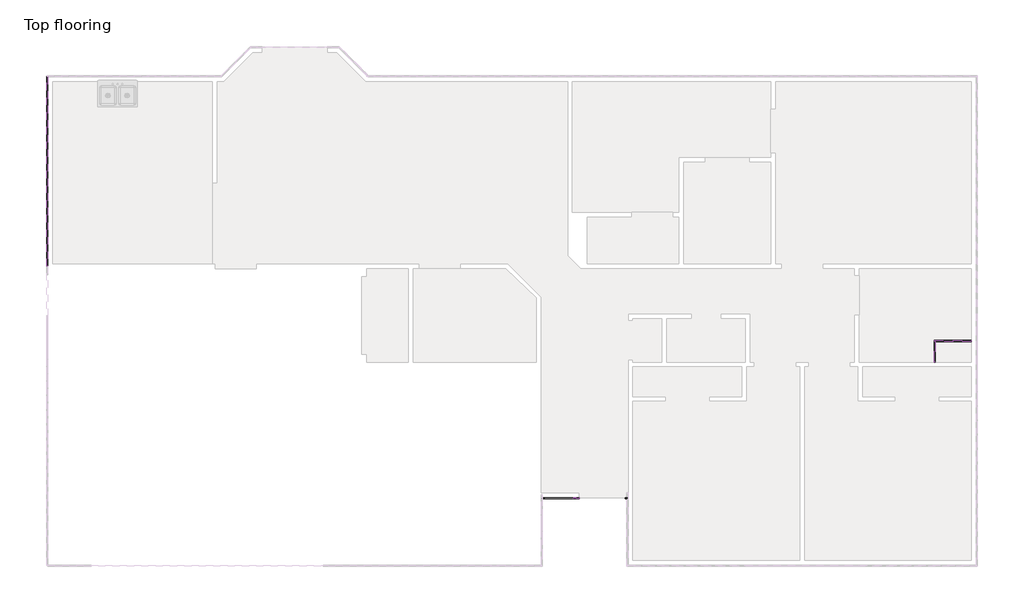
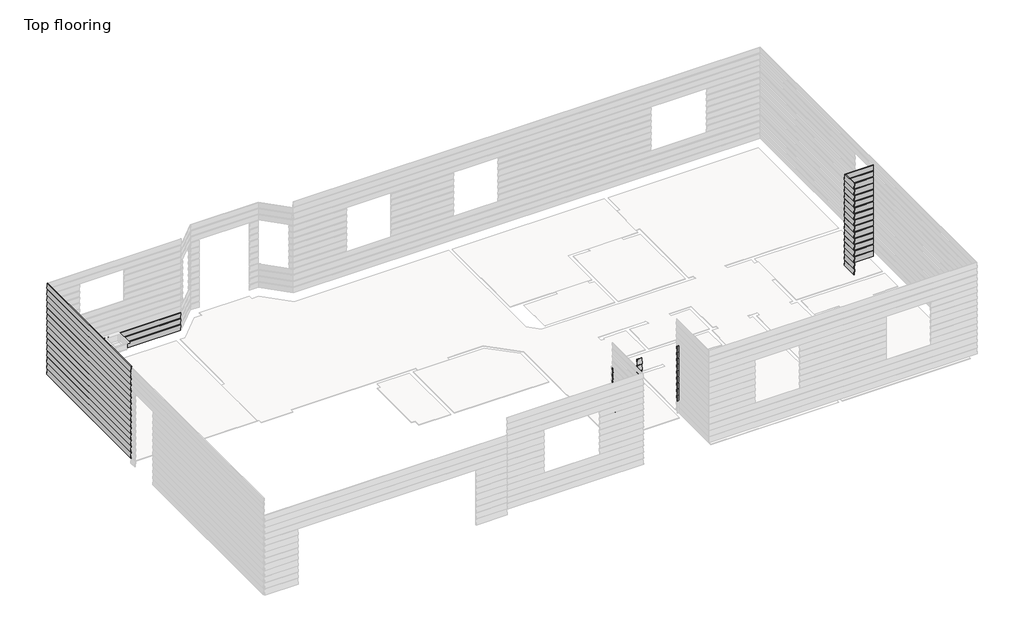
# One storey, part 3 of 5: 57 proxies.
"""IFC4 building model written with IfcOpenShell, lengths in millimetres."""

from ifc_helpers import new_model, si_unit, frame, origin, place, context, project, spatial, polyline, outline, extrude, faceted_brep, element, save

model = new_model("IFC4")

# Units and contexts
model_context = context("Model", 3, world=origin())
ifc_project = project(units=[si_unit("LENGTHUNIT", "METRE", prefix="MILLI")], contexts=[model_context])

# Site, building, storey
site = spatial("IfcSite", under=ifc_project)
building = spatial("IfcBuilding", under=site)
storey = spatial("IfcBuildingStorey", under=building, Name="Top flooring", Elevation=12.7)

# Proxies
placement = place(None, origin())
element("IfcBuildingElementProxy", 1, Name="Wall Sweeps", at=placement, inside=storey, context=model_context, shape_type="Brep", body=[
    faceted_brep([(-17825.3509195, 5231.8645018, 179.3151454), (-17811.1755052, 5217.6890875, 338.6859634), (-17801.214829, 5207.7284114, 337.8), (-17815.3902433, 5221.9038257, 178.429182), (-17825.3509195, 1226.2784114, 179.3151454), (-17815.3902433, 1226.2784114, 178.429182), (-17801.214829, 1226.2784114, 337.8), (-17811.1755052, 1226.2784114, 338.6859634)], [[[0, 1, 2, 3]], [[4, 5, 6, 7]], [[1, 0, 4, 7]], [[2, 1, 7, 6]], [[3, 2, 6, 5]], [[0, 3, 5, 4]]]),
])
element("IfcBuildingElementProxy", 2, Name="Wall Sweeps", at=placement, inside=storey, context=model_context, shape_type="Brep", body=[
    faceted_brep([(-17825.3509195, 5231.8645018, 357.1151454), (-17811.1755052, 5217.6890875, 516.4859634), (-17801.214829, 5207.7284114, 515.6), (-17815.3902433, 5221.9038257, 356.229182), (-17825.3509195, 1226.2784114, 357.1151454), (-17815.3902433, 1226.2784114, 356.229182), (-17801.214829, 1226.2784114, 515.6), (-17811.1755052, 1226.2784114, 516.4859634)], [[[0, 1, 2, 3]], [[4, 5, 6, 7]], [[1, 0, 4, 7]], [[2, 1, 7, 6]], [[3, 2, 6, 5]], [[0, 3, 5, 4]]]),
])
element("IfcBuildingElementProxy", 3, Name="Wall Sweeps", at=placement, inside=storey, context=model_context, shape_type="Brep", body=[
    faceted_brep([(-17825.3509195, 5231.8645018, 534.9151454), (-17811.1755052, 5217.6890875, 694.2859634), (-17801.214829, 5207.7284114, 693.4), (-17815.3902433, 5221.9038257, 534.029182), (-17825.3509195, 1226.2784114, 534.9151454), (-17815.3902433, 1226.2784114, 534.029182), (-17801.214829, 1226.2784114, 693.4), (-17811.1755052, 1226.2784114, 694.2859634)], [[[0, 1, 2, 3]], [[4, 5, 6, 7]], [[1, 0, 4, 7]], [[2, 1, 7, 6]], [[3, 2, 6, 5]], [[0, 3, 5, 4]]]),
])
element("IfcBuildingElementProxy", 4, Name="Wall Sweeps", at=placement, inside=storey, context=model_context, shape_type="Brep", body=[
    faceted_brep([(-17825.3509195, 5231.8645018, 712.7151454), (-17811.1755052, 5217.6890875, 872.0859634), (-17801.214829, 5207.7284114, 871.2), (-17815.3902433, 5221.9038257, 711.829182), (-17825.3509195, 1226.2784114, 712.7151454), (-17815.3902433, 1226.2784114, 711.829182), (-17801.214829, 1226.2784114, 871.2), (-17811.1755052, 1226.2784114, 872.0859634)], [[[0, 1, 2, 3]], [[4, 5, 6, 7]], [[1, 0, 4, 7]], [[2, 1, 7, 6]], [[3, 2, 6, 5]], [[0, 3, 5, 4]]]),
])
element("IfcBuildingElementProxy", 5, Name="Wall Sweeps", at=placement, inside=storey, context=model_context, shape_type="Brep", body=[
    faceted_brep([(-17825.3509195, 5231.8645018, 890.5151454), (-17811.1755052, 5217.6890875, 1049.8859634), (-17801.214829, 5207.7284114, 1049.0), (-17815.3902433, 5221.9038257, 889.629182), (-17825.3509195, 1226.2784114, 890.5151454), (-17815.3902433, 1226.2784114, 889.629182), (-17801.214829, 1226.2784114, 1049.0), (-17811.1755052, 1226.2784114, 1049.8859634)], [[[0, 1, 2, 3]], [[4, 5, 6, 7]], [[1, 0, 4, 7]], [[2, 1, 7, 6]], [[3, 2, 6, 5]], [[0, 3, 5, 4]]]),
])
element("IfcBuildingElementProxy", 6, Name="Wall Sweeps", at=placement, inside=storey, context=model_context, shape_type="Brep", body=[
    faceted_brep([(-17825.3509195, 5231.8645018, 1068.3151454), (-17811.1755052, 5217.6890875, 1227.6859634), (-17801.214829, 5207.7284114, 1226.8), (-17815.3902433, 5221.9038257, 1067.429182), (-17825.3509195, 1226.2784114, 1068.3151454), (-17815.3902433, 1226.2784114, 1067.429182), (-17801.214829, 1226.2784114, 1226.8), (-17811.1755052, 1226.2784114, 1227.6859634)], [[[0, 1, 2, 3]], [[4, 5, 6, 7]], [[1, 0, 4, 7]], [[2, 1, 7, 6]], [[3, 2, 6, 5]], [[0, 3, 5, 4]]]),
])
element("IfcBuildingElementProxy", 7, Name="Wall Sweeps", at=placement, inside=storey, context=model_context, shape_type="Brep", body=[
    faceted_brep([(-17825.3509195, 5231.8645018, 1246.1151454), (-17811.1755052, 5217.6890875, 1405.4859634), (-17801.214829, 5207.7284114, 1404.6), (-17815.3902433, 5221.9038257, 1245.229182), (-17825.3509195, 1226.2784114, 1246.1151454), (-17815.3902433, 1226.2784114, 1245.229182), (-17801.214829, 1226.2784114, 1404.6), (-17811.1755052, 1226.2784114, 1405.4859634)], [[[0, 1, 2, 3]], [[4, 5, 6, 7]], [[1, 0, 4, 7]], [[2, 1, 7, 6]], [[3, 2, 6, 5]], [[0, 3, 5, 4]]]),
])
element("IfcBuildingElementProxy", 8, Name="Wall Sweeps", at=placement, inside=storey, context=model_context, shape_type="Brep", body=[
    faceted_brep([(-17825.3509195, 5231.8645018, 1423.9151454), (-17811.1755052, 5217.6890875, 1583.2859634), (-17801.214829, 5207.7284114, 1582.4), (-17815.3902433, 5221.9038257, 1423.029182), (-17825.3509195, 1226.2784114, 1423.9151454), (-17815.3902433, 1226.2784114, 1423.029182), (-17801.214829, 1226.2784114, 1582.4), (-17811.1755052, 1226.2784114, 1583.2859634)], [[[0, 1, 2, 3]], [[4, 5, 6, 7]], [[1, 0, 4, 7]], [[2, 1, 7, 6]], [[3, 2, 6, 5]], [[0, 3, 5, 4]]]),
])
element("IfcBuildingElementProxy", 9, Name="Wall Sweeps", at=placement, inside=storey, context=model_context, shape_type="Brep", body=[
    faceted_brep([(-17825.3509195, 5231.8645018, 1601.7151454), (-17811.1755052, 5217.6890875, 1761.0859634), (-17801.214829, 5207.7284114, 1760.2), (-17815.3902433, 5221.9038257, 1600.829182), (-17825.3509195, 1226.2784114, 1601.7151454), (-17815.3902433, 1226.2784114, 1600.829182), (-17801.214829, 1226.2784114, 1760.2), (-17811.1755052, 1226.2784114, 1761.0859634)], [[[0, 1, 2, 3]], [[4, 5, 6, 7]], [[1, 0, 4, 7]], [[2, 1, 7, 6]], [[3, 2, 6, 5]], [[0, 3, 5, 4]]]),
])
element("IfcBuildingElementProxy", 10, Name="Wall Sweeps", at=placement, inside=storey, context=model_context, shape_type="Brep", body=[
    faceted_brep([(-17825.3509195, 5231.8645018, 1779.5151454), (-17811.1755052, 5217.6890875, 1938.8859634), (-17801.214829, 5207.7284114, 1938.0), (-17815.3902433, 5221.9038257, 1778.629182), (-17825.3509195, 1226.2784114, 1779.5151454), (-17815.3902433, 1226.2784114, 1778.629182), (-17801.214829, 1226.2784114, 1938.0), (-17811.1755052, 1226.2784114, 1938.8859634)], [[[0, 1, 2, 3]], [[4, 5, 6, 7]], [[1, 0, 4, 7]], [[2, 1, 7, 6]], [[3, 2, 6, 5]], [[0, 3, 5, 4]]]),
])
element("IfcBuildingElementProxy", 11, Name="Wall Sweeps", at=placement, inside=storey, context=model_context, shape_type="Brep", body=[
    faceted_brep([(-17825.3509195, 5231.8645018, 1957.3151454), (-17811.1755052, 5217.6890875, 2116.6859634), (-17801.214829, 5207.7284114, 2115.8), (-17815.3902433, 5221.9038257, 1956.429182), (-17825.3509195, 1226.2784114, 1957.3151454), (-17815.3902433, 1226.2784114, 1956.429182), (-17801.214829, 1226.2784114, 2115.8), (-17811.1755052, 1226.2784114, 2116.6859634)], [[[0, 1, 2, 3]], [[4, 5, 6, 7]], [[1, 0, 4, 7]], [[2, 1, 7, 6]], [[3, 2, 6, 5]], [[0, 3, 5, 4]]]),
])
element("IfcBuildingElementProxy", 12, Name="Wall Sweeps", at=placement, inside=storey, context=model_context, shape_type="Brep", body=[
    faceted_brep([(-17825.3509195, 5231.8645018, 2135.1151454), (-17811.1755052, 5217.6890875, 2294.4859634), (-17801.214829, 5207.7284114, 2293.6), (-17815.3902433, 5221.9038257, 2134.229182), (-17825.3509195, 1226.2784114, 2135.1151454), (-17815.3902433, 1226.2784114, 2134.229182), (-17801.214829, 1226.2784114, 2293.6), (-17811.1755052, 1226.2784114, 2294.4859634)], [[[0, 1, 2, 3]], [[4, 5, 6, 7]], [[1, 0, 4, 7]], [[2, 1, 7, 6]], [[3, 2, 6, 5]], [[0, 3, 5, 4]]]),
])
element("IfcBuildingElementProxy", 13, Name="Wall Sweeps", at=placement, inside=storey, context=model_context, shape_type="Brep", body=[
    faceted_brep([(-17825.3509195, 5231.8645018, 179.3151454), (-17815.3902433, 5221.9038257, 178.429182), (-17801.214829, 5207.7284114, 337.8), (-17811.1755052, 5217.6890875, 338.6859634), (-14153.612325, 5231.8645018, 179.3151454), (-14147.7406762, 5217.6890875, 338.6859634), (-14143.614829, 5207.7284114, 337.8), (-14149.4864779, 5221.9038257, 178.429182)], [[[0, 1, 2, 3]], [[4, 5, 6, 7]], [[1, 0, 4, 7]], [[2, 1, 7, 6]], [[3, 2, 6, 5]], [[0, 3, 5, 4]]]),
])
element("IfcBuildingElementProxy", 14, Name="Wall Sweeps", at=placement, inside=storey, context=model_context, shape_type="Brep", body=[
    faceted_brep([(-17825.3509195, 5231.8645018, 357.1151454), (-17815.3902433, 5221.9038257, 356.229182), (-17801.214829, 5207.7284114, 515.6), (-17811.1755052, 5217.6890875, 516.4859634), (-14153.612325, 5231.8645018, 357.1151454), (-14147.7406762, 5217.6890875, 516.4859634), (-14143.614829, 5207.7284114, 515.6), (-14149.4864779, 5221.9038257, 356.229182)], [[[0, 1, 2, 3]], [[4, 5, 6, 7]], [[1, 0, 4, 7]], [[2, 1, 7, 6]], [[3, 2, 6, 5]], [[0, 3, 5, 4]]]),
])
element("IfcBuildingElementProxy", 15, Name="Wall Sweeps", at=placement, inside=storey, context=model_context, shape_type="Brep", body=[
    faceted_brep([(-17825.3509195, 5231.8645018, 534.9151454), (-17815.3902433, 5221.9038257, 534.029182), (-17801.214829, 5207.7284114, 693.4), (-17811.1755052, 5217.6890875, 694.2859634), (-14153.612325, 5231.8645018, 534.9151454), (-14147.7406762, 5217.6890875, 694.2859634), (-14143.614829, 5207.7284114, 693.4), (-14149.4864779, 5221.9038257, 534.029182)], [[[0, 1, 2, 3]], [[4, 5, 6, 7]], [[1, 0, 4, 7]], [[2, 1, 7, 6]], [[3, 2, 6, 5]], [[0, 3, 5, 4]]]),
])
element("IfcBuildingElementProxy", 16, Name="Wall Sweeps", at=placement, inside=storey, context=model_context, shape_type="SweptSolid", body=[
    extrude(outline(polyline([(0.0, -10.0), (0.0, 0.0), (63.9, 0.0), (63.9, -10.0), (0.0, -10.0)])), frame((-5673.114829, -3645.6470029, 534.029182), z_axis=(0.0, 0.08859633935570814, 0.9960676124906221), x_axis=(1.0, 0.0, 0.0)), (0.0, 0.0, 1.0), 160.0),
    extrude(outline(polyline([(0.0, -10.0), (0.0, 0.0), (800.5, 0.0), (800.5, -10.0), (0.0, -10.0)])), frame((-7438.014829, -3645.6470029, 534.029182), z_axis=(0.0, 0.08859633935570814, 0.9960676124906221), x_axis=(1.0, 0.0, 0.0)), (0.0, 0.0, 1.0), 160.0),
])
element("IfcBuildingElementProxy", 17, Name="Wall Sweeps", at=placement, inside=storey, context=model_context, shape_type="SweptSolid", body=[
    extrude(outline(polyline([(0.0, -10.0), (0.0, 0.0), (63.9, 0.0), (63.9, -10.0), (0.0, -10.0)])), frame((-5673.114829, -3645.6470029, 711.829182), z_axis=(0.0, 0.08859633935570814, 0.9960676124906221), x_axis=(1.0, 0.0, 0.0)), (0.0, 0.0, 1.0), 160.0),
    extrude(outline(polyline([(0.0, -10.0), (0.0, 0.0), (800.5, 0.0), (800.5, -10.0), (0.0, -10.0)])), frame((-7438.014829, -3645.6470029, 711.829182), z_axis=(0.0, 0.08859633935570814, 0.9960676124906221), x_axis=(1.0, 0.0, 0.0)), (0.0, 0.0, 1.0), 160.0),
])
element("IfcBuildingElementProxy", 18, Name="Wall Sweeps", at=placement, inside=storey, context=model_context, shape_type="SweptSolid", body=[
    extrude(outline(polyline([(0.0, -10.0), (0.0, 0.0), (63.9, 0.0), (63.9, -10.0), (0.0, -10.0)])), frame((-5673.114829, -3645.6470029, 889.629182), z_axis=(0.0, 0.08859633935570814, 0.9960676124906221), x_axis=(1.0, 0.0, 0.0)), (0.0, 0.0, 1.0), 160.0),
    extrude(outline(polyline([(0.0, -10.0), (0.0, 0.0), (127.4, 0.0), (127.4, -10.0), (0.0, -10.0)])), frame((-6764.914829, -3645.6470029, 889.629182), z_axis=(0.0, 0.08859633935570814, 0.9960676124906221), x_axis=(1.0, 0.0, 0.0)), (0.0, 0.0, 1.0), 160.0),
    extrude(outline(polyline([(0.0, -10.0), (0.0, 0.0), (63.5, 0.0), (63.5, -10.0), (0.0, -10.0)])), frame((-7438.014829, -3645.6470029, 889.629182), z_axis=(0.0, 0.08859633935570814, 0.9960676124906221), x_axis=(1.0, 0.0, 0.0)), (0.0, 0.0, 1.0), 160.0),
])
element("IfcBuildingElementProxy", 19, Name="Wall Sweeps", at=placement, inside=storey, context=model_context, shape_type="SweptSolid", body=[
    extrude(outline(polyline([(0.0, -10.0), (0.0, 0.0), (63.9, 0.0), (63.9, -10.0), (0.0, -10.0)])), frame((-5673.114829, -3645.6470029, 1067.429182), z_axis=(0.0, 0.08859633935570814, 0.9960676124906221), x_axis=(1.0, 0.0, 0.0)), (0.0, 0.0, 1.0), 160.0),
    extrude(outline(polyline([(0.0, -10.0), (0.0, 0.0), (127.4, 0.0), (127.4, -10.0), (0.0, -10.0)])), frame((-6764.914829, -3645.6470029, 1067.429182), z_axis=(0.0, 0.08859633935570814, 0.9960676124906221), x_axis=(1.0, 0.0, 0.0)), (0.0, 0.0, 1.0), 160.0),
    extrude(outline(polyline([(0.0, -10.0), (0.0, 0.0), (63.5, 0.0), (63.5, -10.0), (0.0, -10.0)])), frame((-7438.014829, -3645.6470029, 1067.429182), z_axis=(0.0, 0.08859633935570814, 0.9960676124906221), x_axis=(1.0, 0.0, 0.0)), (0.0, 0.0, 1.0), 160.0),
])
element("IfcBuildingElementProxy", 20, Name="Wall Sweeps", at=placement, inside=storey, context=model_context, shape_type="SweptSolid", body=[
    extrude(outline(polyline([(0.0, -10.0), (0.0, 0.0), (63.9, 0.0), (63.9, -10.0), (0.0, -10.0)])), frame((-5673.114829, -3645.6470029, 1245.229182), z_axis=(0.0, 0.08859633935570814, 0.9960676124906221), x_axis=(1.0, 0.0, 0.0)), (0.0, 0.0, 1.0), 160.0),
    extrude(outline(polyline([(0.0, -10.0), (0.0, 0.0), (127.4, 0.0), (127.4, -10.0), (0.0, -10.0)])), frame((-6764.914829, -3645.6470029, 1245.229182), z_axis=(0.0, 0.08859633935570814, 0.9960676124906221), x_axis=(1.0, 0.0, 0.0)), (0.0, 0.0, 1.0), 160.0),
    extrude(outline(polyline([(0.0, -10.0), (0.0, 0.0), (63.5, 0.0), (63.5, -10.0), (0.0, -10.0)])), frame((-7438.014829, -3645.6470029, 1245.229182), z_axis=(0.0, 0.08859633935570814, 0.9960676124906221), x_axis=(1.0, 0.0, 0.0)), (0.0, 0.0, 1.0), 160.0),
])
element("IfcBuildingElementProxy", 21, Name="Wall Sweeps", at=placement, inside=storey, context=model_context, shape_type="SweptSolid", body=[
    extrude(outline(polyline([(0.0, -10.0), (0.0, 0.0), (63.9, 0.0), (63.9, -10.0), (0.0, -10.0)])), frame((-5673.114829, -3645.6470029, 1423.029182), z_axis=(0.0, 0.08859633935570814, 0.9960676124906221), x_axis=(1.0, 0.0, 0.0)), (0.0, 0.0, 1.0), 160.0),
    extrude(outline(polyline([(0.0, -10.0), (0.0, 0.0), (127.4, 0.0), (127.4, -10.0), (0.0, -10.0)])), frame((-6764.914829, -3645.6470029, 1423.029182), z_axis=(0.0, 0.08859633935570814, 0.9960676124906221), x_axis=(1.0, 0.0, 0.0)), (0.0, 0.0, 1.0), 160.0),
    extrude(outline(polyline([(0.0, -10.0), (0.0, 0.0), (63.5, 0.0), (63.5, -10.0), (0.0, -10.0)])), frame((-7438.014829, -3645.6470029, 1423.029182), z_axis=(0.0, 0.08859633935570814, 0.9960676124906221), x_axis=(1.0, 0.0, 0.0)), (0.0, 0.0, 1.0), 160.0),
])
element("IfcBuildingElementProxy", 22, Name="Wall Sweeps", at=placement, inside=storey, context=model_context, shape_type="SweptSolid", body=[
    extrude(outline(polyline([(0.0, -10.0), (0.0, 0.0), (63.9, 0.0), (63.9, -10.0), (0.0, -10.0)])), frame((-5673.114829, -3645.6470029, 1600.829182), z_axis=(0.0, 0.08859633935570814, 0.9960676124906221), x_axis=(1.0, 0.0, 0.0)), (0.0, 0.0, 1.0), 160.0),
    extrude(outline(polyline([(0.0, -10.0), (0.0, 0.0), (127.4, 0.0), (127.4, -10.0), (0.0, -10.0)])), frame((-6764.914829, -3645.6470029, 1600.829182), z_axis=(0.0, 0.08859633935570814, 0.9960676124906221), x_axis=(1.0, 0.0, 0.0)), (0.0, 0.0, 1.0), 160.0),
    extrude(outline(polyline([(0.0, -10.0), (0.0, 0.0), (63.5, 0.0), (63.5, -10.0), (0.0, -10.0)])), frame((-7438.014829, -3645.6470029, 1600.829182), z_axis=(0.0, 0.08859633935570814, 0.9960676124906221), x_axis=(1.0, 0.0, 0.0)), (0.0, 0.0, 1.0), 160.0),
])
element("IfcBuildingElementProxy", 23, Name="Wall Sweeps", at=placement, inside=storey, context=model_context, shape_type="SweptSolid", body=[
    extrude(outline(polyline([(0.0, -10.0), (0.0, 0.0), (63.9, 0.0), (63.9, -10.0), (0.0, -10.0)])), frame((-5673.114829, -3645.6470029, 1778.629182), z_axis=(0.0, 0.08859633935570814, 0.9960676124906221), x_axis=(1.0, 0.0, 0.0)), (0.0, 0.0, 1.0), 160.0),
    extrude(outline(polyline([(0.0, -10.0), (0.0, 0.0), (127.4, 0.0), (127.4, -10.0), (0.0, -10.0)])), frame((-6764.914829, -3645.6470029, 1778.629182), z_axis=(0.0, 0.08859633935570814, 0.9960676124906221), x_axis=(1.0, 0.0, 0.0)), (0.0, 0.0, 1.0), 160.0),
    extrude(outline(polyline([(0.0, -10.0), (0.0, 0.0), (63.5, 0.0), (63.5, -10.0), (0.0, -10.0)])), frame((-7438.014829, -3645.6470029, 1778.629182), z_axis=(0.0, 0.08859633935570814, 0.9960676124906221), x_axis=(1.0, 0.0, 0.0)), (0.0, 0.0, 1.0), 160.0),
])
element("IfcBuildingElementProxy", 24, Name="Wall Sweeps", at=placement, inside=storey, context=model_context, shape_type="SweptSolid", body=[
    extrude(outline(polyline([(0.0, -10.0), (0.0, 0.0), (63.9, 0.0), (63.9, -10.0), (0.0, -10.0)])), frame((-5673.114829, -3645.6470029, 1956.429182), z_axis=(0.0, 0.08859633935570814, 0.9960676124906221), x_axis=(1.0, 0.0, 0.0)), (0.0, 0.0, 1.0), 160.0),
    extrude(outline(polyline([(0.0, -10.0), (0.0, 0.0), (127.4, 0.0), (127.4, -10.0), (0.0, -10.0)])), frame((-6764.914829, -3645.6470029, 1956.429182), z_axis=(0.0, 0.08859633935570814, 0.9960676124906221), x_axis=(1.0, 0.0, 0.0)), (0.0, 0.0, 1.0), 160.0),
    extrude(outline(polyline([(0.0, -10.0), (0.0, 0.0), (63.5, 0.0), (63.5, -10.0), (0.0, -10.0)])), frame((-7438.014829, -3645.6470029, 1956.429182), z_axis=(0.0, 0.08859633935570814, 0.9960676124906221), x_axis=(1.0, 0.0, 0.0)), (0.0, 0.0, 1.0), 160.0),
])
element("IfcBuildingElementProxy", 25, Name="Wall Sweeps", at=placement, inside=storey, context=model_context, shape_type="Brep", body=[
    faceted_brep([(1604.385171, -330.7354982, 179.3151454), (1604.385171, -344.9109125, 338.6859634), (1604.385171, -354.8715886, 337.8), (1604.385171, -340.6961743, 178.429182), (818.2490805, -330.7354982, 179.3151454), (828.2097567, -340.6961743, 178.429182), (842.385171, -354.8715886, 337.8), (832.4244948, -344.9109125, 338.6859634)], [[[0, 1, 2, 3]], [[4, 5, 6, 7]], [[1, 0, 4, 7]], [[2, 1, 7, 6]], [[3, 2, 6, 5]], [[0, 3, 5, 4]]]),
])
element("IfcBuildingElementProxy", 26, Name="Wall Sweeps", at=placement, inside=storey, context=model_context, shape_type="Brep", body=[
    faceted_brep([(1604.385171, -330.7354982, 357.1151454), (1604.385171, -344.9109125, 516.4859634), (1604.385171, -354.8715886, 515.6), (1604.385171, -340.6961743, 356.229182), (818.2490805, -330.7354982, 357.1151454), (828.2097567, -340.6961743, 356.229182), (842.385171, -354.8715886, 515.6), (832.4244948, -344.9109125, 516.4859634)], [[[0, 1, 2, 3]], [[4, 5, 6, 7]], [[1, 0, 4, 7]], [[2, 1, 7, 6]], [[3, 2, 6, 5]], [[0, 3, 5, 4]]]),
])
element("IfcBuildingElementProxy", 27, Name="Wall Sweeps", at=placement, inside=storey, context=model_context, shape_type="Brep", body=[
    faceted_brep([(1604.385171, -330.7354982, 534.9151454), (1604.385171, -344.9109125, 694.2859634), (1604.385171, -354.8715886, 693.4), (1604.385171, -340.6961743, 534.029182), (818.2490805, -330.7354982, 534.9151454), (828.2097567, -340.6961743, 534.029182), (842.385171, -354.8715886, 693.4), (832.4244948, -344.9109125, 694.2859634)], [[[0, 1, 2, 3]], [[4, 5, 6, 7]], [[1, 0, 4, 7]], [[2, 1, 7, 6]], [[3, 2, 6, 5]], [[0, 3, 5, 4]]]),
])
element("IfcBuildingElementProxy", 28, Name="Wall Sweeps", at=placement, inside=storey, context=model_context, shape_type="Brep", body=[
    faceted_brep([(1604.385171, -330.7354982, 712.7151454), (1604.385171, -344.9109125, 872.0859634), (1604.385171, -354.8715886, 871.2), (1604.385171, -340.6961743, 711.829182), (818.2490805, -330.7354982, 712.7151454), (828.2097567, -340.6961743, 711.829182), (842.385171, -354.8715886, 871.2), (832.4244948, -344.9109125, 872.0859634)], [[[0, 1, 2, 3]], [[4, 5, 6, 7]], [[1, 0, 4, 7]], [[2, 1, 7, 6]], [[3, 2, 6, 5]], [[0, 3, 5, 4]]]),
])
element("IfcBuildingElementProxy", 29, Name="Wall Sweeps", at=placement, inside=storey, context=model_context, shape_type="Brep", body=[
    faceted_brep([(1604.385171, -330.7354982, 890.5151454), (1604.385171, -344.9109125, 1049.8859634), (1604.385171, -354.8715886, 1049.0), (1604.385171, -340.6961743, 889.629182), (818.2490805, -330.7354982, 890.5151454), (828.2097567, -340.6961743, 889.629182), (842.385171, -354.8715886, 1049.0), (832.4244948, -344.9109125, 1049.8859634)], [[[0, 1, 2, 3]], [[4, 5, 6, 7]], [[1, 0, 4, 7]], [[2, 1, 7, 6]], [[3, 2, 6, 5]], [[0, 3, 5, 4]]]),
])
element("IfcBuildingElementProxy", 30, Name="Wall Sweeps", at=placement, inside=storey, context=model_context, shape_type="Brep", body=[
    faceted_brep([(1604.385171, -330.7354982, 1068.3151454), (1604.385171, -344.9109125, 1227.6859634), (1604.385171, -354.8715886, 1226.8), (1604.385171, -340.6961743, 1067.429182), (818.2490805, -330.7354982, 1068.3151454), (828.2097567, -340.6961743, 1067.429182), (842.385171, -354.8715886, 1226.8), (832.4244948, -344.9109125, 1227.6859634)], [[[0, 1, 2, 3]], [[4, 5, 6, 7]], [[1, 0, 4, 7]], [[2, 1, 7, 6]], [[3, 2, 6, 5]], [[0, 3, 5, 4]]]),
])
element("IfcBuildingElementProxy", 31, Name="Wall Sweeps", at=placement, inside=storey, context=model_context, shape_type="Brep", body=[
    faceted_brep([(1604.385171, -330.7354982, 1246.1151454), (1604.385171, -344.9109125, 1405.4859634), (1604.385171, -354.8715886, 1404.6), (1604.385171, -340.6961743, 1245.229182), (818.2490805, -330.7354982, 1246.1151454), (828.2097567, -340.6961743, 1245.229182), (842.385171, -354.8715886, 1404.6), (832.4244948, -344.9109125, 1405.4859634)], [[[0, 1, 2, 3]], [[4, 5, 6, 7]], [[1, 0, 4, 7]], [[2, 1, 7, 6]], [[3, 2, 6, 5]], [[0, 3, 5, 4]]]),
])
element("IfcBuildingElementProxy", 32, Name="Wall Sweeps", at=placement, inside=storey, context=model_context, shape_type="Brep", body=[
    faceted_brep([(1604.385171, -330.7354982, 1423.9151454), (1604.385171, -344.9109125, 1583.2859634), (1604.385171, -354.8715886, 1582.4), (1604.385171, -340.6961743, 1423.029182), (818.2490805, -330.7354982, 1423.9151454), (828.2097567, -340.6961743, 1423.029182), (842.385171, -354.8715886, 1582.4), (832.4244948, -344.9109125, 1583.2859634)], [[[0, 1, 2, 3]], [[4, 5, 6, 7]], [[1, 0, 4, 7]], [[2, 1, 7, 6]], [[3, 2, 6, 5]], [[0, 3, 5, 4]]]),
])
element("IfcBuildingElementProxy", 33, Name="Wall Sweeps", at=placement, inside=storey, context=model_context, shape_type="Brep", body=[
    faceted_brep([(1604.385171, -330.7354982, 1601.7151454), (1604.385171, -344.9109125, 1761.0859634), (1604.385171, -354.8715886, 1760.2), (1604.385171, -340.6961743, 1600.829182), (818.2490805, -330.7354982, 1601.7151454), (828.2097567, -340.6961743, 1600.829182), (842.385171, -354.8715886, 1760.2), (832.4244948, -344.9109125, 1761.0859634)], [[[0, 1, 2, 3]], [[4, 5, 6, 7]], [[1, 0, 4, 7]], [[2, 1, 7, 6]], [[3, 2, 6, 5]], [[0, 3, 5, 4]]]),
])
element("IfcBuildingElementProxy", 34, Name="Wall Sweeps", at=placement, inside=storey, context=model_context, shape_type="Brep", body=[
    faceted_brep([(1604.385171, -330.7354982, 1779.5151454), (1604.385171, -344.9109125, 1938.8859634), (1604.385171, -354.8715886, 1938.0), (1604.385171, -340.6961743, 1778.629182), (818.2490805, -330.7354982, 1779.5151454), (828.2097567, -340.6961743, 1778.629182), (842.385171, -354.8715886, 1938.0), (832.4244948, -344.9109125, 1938.8859634)], [[[0, 1, 2, 3]], [[4, 5, 6, 7]], [[1, 0, 4, 7]], [[2, 1, 7, 6]], [[3, 2, 6, 5]], [[0, 3, 5, 4]]]),
])
element("IfcBuildingElementProxy", 35, Name="Wall Sweeps", at=placement, inside=storey, context=model_context, shape_type="Brep", body=[
    faceted_brep([(1604.385171, -330.7354982, 1957.3151454), (1604.385171, -344.9109125, 2116.6859634), (1604.385171, -354.8715886, 2115.8), (1604.385171, -340.6961743, 1956.429182), (818.2490805, -330.7354982, 1957.3151454), (828.2097567, -340.6961743, 1956.429182), (842.385171, -354.8715886, 2115.8), (832.4244948, -344.9109125, 2116.6859634)], [[[0, 1, 2, 3]], [[4, 5, 6, 7]], [[1, 0, 4, 7]], [[2, 1, 7, 6]], [[3, 2, 6, 5]], [[0, 3, 5, 4]]]),
])
element("IfcBuildingElementProxy", 36, Name="Wall Sweeps", at=placement, inside=storey, context=model_context, shape_type="Brep", body=[
    faceted_brep([(1604.385171, -330.7354982, 2135.1151454), (1604.385171, -344.9109125, 2294.4859634), (1604.385171, -354.8715886, 2293.6), (1604.385171, -340.6961743, 2134.229182), (818.2490805, -330.7354982, 2135.1151454), (828.2097567, -340.6961743, 2134.229182), (842.385171, -354.8715886, 2293.6), (832.4244948, -344.9109125, 2294.4859634)], [[[0, 1, 2, 3]], [[4, 5, 6, 7]], [[1, 0, 4, 7]], [[2, 1, 7, 6]], [[3, 2, 6, 5]], [[0, 3, 5, 4]]]),
])
element("IfcBuildingElementProxy", 37, Name="Wall Sweeps", at=placement, inside=storey, context=model_context, shape_type="Brep", body=[
    faceted_brep([(1604.385171, -330.7354982, 2312.9151454), (1604.385171, -344.9109125, 2472.2859634), (1604.385171, -354.8715886, 2471.4), (1604.385171, -340.6961743, 2312.029182), (818.2490805, -330.7354982, 2312.9151454), (828.2097567, -340.6961743, 2312.029182), (842.385171, -354.8715886, 2471.4), (832.4244948, -344.9109125, 2472.2859634)], [[[0, 1, 2, 3]], [[4, 5, 6, 7]], [[1, 0, 4, 7]], [[2, 1, 7, 6]], [[3, 2, 6, 5]], [[0, 3, 5, 4]]]),
])
element("IfcBuildingElementProxy", 38, Name="Wall Sweeps", at=placement, inside=storey, context=model_context, shape_type="Brep", body=[
    faceted_brep([(1604.385171, -330.7354982, 2490.7151454), (1604.385171, -344.9109125, 2650.0859634), (1604.385171, -354.8715886, 2649.2), (1604.385171, -340.6961743, 2489.829182), (818.2490805, -330.7354982, 2490.7151454), (828.2097567, -340.6961743, 2489.829182), (842.385171, -354.8715886, 2649.2), (832.4244948, -344.9109125, 2650.0859634)], [[[0, 1, 2, 3]], [[4, 5, 6, 7]], [[1, 0, 4, 7]], [[2, 1, 7, 6]], [[3, 2, 6, 5]], [[0, 3, 5, 4]]]),
])
element("IfcBuildingElementProxy", 39, Name="Wall Sweeps", at=placement, inside=storey, context=model_context, shape_type="Brep", body=[
    faceted_brep([(1604.385171, -330.7354982, 2668.5151454), (1604.385171, -344.9109125, 2827.8859634), (1604.385171, -354.8715886, 2827.0), (1604.385171, -340.6961743, 2667.629182), (818.2490805, -330.7354982, 2668.5151454), (828.2097567, -340.6961743, 2667.629182), (842.385171, -354.8715886, 2827.0), (832.4244948, -344.9109125, 2827.8859634)], [[[0, 1, 2, 3]], [[4, 5, 6, 7]], [[1, 0, 4, 7]], [[2, 1, 7, 6]], [[3, 2, 6, 5]], [[0, 3, 5, 4]]]),
])
element("IfcBuildingElementProxy", 40, Name="Wall Sweeps", at=placement, inside=storey, context=model_context, shape_type="Brep", body=[
    faceted_brep([(818.2490805, -330.7354982, 179.3151454), (832.4244948, -344.9109125, 338.6859634), (842.385171, -354.8715886, 337.8), (828.2097567, -340.6961743, 178.429182), (818.2490805, -786.6715886, 179.3151454), (828.2097567, -786.6715886, 178.429182), (842.385171, -786.6715886, 337.8), (832.4244948, -786.6715886, 338.6859634)], [[[0, 1, 2, 3]], [[4, 5, 6, 7]], [[1, 0, 4, 7]], [[2, 1, 7, 6]], [[3, 2, 6, 5]], [[0, 3, 5, 4]]]),
])
element("IfcBuildingElementProxy", 41, Name="Wall Sweeps", at=placement, inside=storey, context=model_context, shape_type="Brep", body=[
    faceted_brep([(818.2490805, -330.7354982, 357.1151454), (832.4244948, -344.9109125, 516.4859634), (842.385171, -354.8715886, 515.6), (828.2097567, -340.6961743, 356.229182), (818.2490805, -786.6715886, 357.1151454), (828.2097567, -786.6715886, 356.229182), (842.385171, -786.6715886, 515.6), (832.4244948, -786.6715886, 516.4859634)], [[[0, 1, 2, 3]], [[4, 5, 6, 7]], [[1, 0, 4, 7]], [[2, 1, 7, 6]], [[3, 2, 6, 5]], [[0, 3, 5, 4]]]),
])
element("IfcBuildingElementProxy", 42, Name="Wall Sweeps", at=placement, inside=storey, context=model_context, shape_type="Brep", body=[
    faceted_brep([(818.2490805, -330.7354982, 534.9151454), (832.4244948, -344.9109125, 694.2859634), (842.385171, -354.8715886, 693.4), (828.2097567, -340.6961743, 534.029182), (818.2490805, -786.6715886, 534.9151454), (828.2097567, -786.6715886, 534.029182), (842.385171, -786.6715886, 693.4), (832.4244948, -786.6715886, 694.2859634)], [[[0, 1, 2, 3]], [[4, 5, 6, 7]], [[1, 0, 4, 7]], [[2, 1, 7, 6]], [[3, 2, 6, 5]], [[0, 3, 5, 4]]]),
])
element("IfcBuildingElementProxy", 43, Name="Wall Sweeps", at=placement, inside=storey, context=model_context, shape_type="Brep", body=[
    faceted_brep([(818.2490805, -330.7354982, 712.7151454), (832.4244948, -344.9109125, 872.0859634), (842.385171, -354.8715886, 871.2), (828.2097567, -340.6961743, 711.829182), (818.2490805, -786.6715886, 712.7151454), (828.2097567, -786.6715886, 711.829182), (842.385171, -786.6715886, 871.2), (832.4244948, -786.6715886, 872.0859634)], [[[0, 1, 2, 3]], [[4, 5, 6, 7]], [[1, 0, 4, 7]], [[2, 1, 7, 6]], [[3, 2, 6, 5]], [[0, 3, 5, 4]]]),
])
element("IfcBuildingElementProxy", 44, Name="Wall Sweeps", at=placement, inside=storey, context=model_context, shape_type="Brep", body=[
    faceted_brep([(818.2490805, -330.7354982, 890.5151454), (832.4244948, -344.9109125, 1049.8859634), (842.385171, -354.8715886, 1049.0), (828.2097567, -340.6961743, 889.629182), (818.2490805, -786.6715886, 890.5151454), (828.2097567, -786.6715886, 889.629182), (842.385171, -786.6715886, 1049.0), (832.4244948, -786.6715886, 1049.8859634)], [[[0, 1, 2, 3]], [[4, 5, 6, 7]], [[1, 0, 4, 7]], [[2, 1, 7, 6]], [[3, 2, 6, 5]], [[0, 3, 5, 4]]]),
])
element("IfcBuildingElementProxy", 45, Name="Wall Sweeps", at=placement, inside=storey, context=model_context, shape_type="Brep", body=[
    faceted_brep([(818.2490805, -330.7354982, 1068.3151454), (832.4244948, -344.9109125, 1227.6859634), (842.385171, -354.8715886, 1226.8), (828.2097567, -340.6961743, 1067.429182), (818.2490805, -786.6715886, 1068.3151454), (828.2097567, -786.6715886, 1067.429182), (842.385171, -786.6715886, 1226.8), (832.4244948, -786.6715886, 1227.6859634)], [[[0, 1, 2, 3]], [[4, 5, 6, 7]], [[1, 0, 4, 7]], [[2, 1, 7, 6]], [[3, 2, 6, 5]], [[0, 3, 5, 4]]]),
])
element("IfcBuildingElementProxy", 46, Name="Wall Sweeps", at=placement, inside=storey, context=model_context, shape_type="Brep", body=[
    faceted_brep([(818.2490805, -330.7354982, 1246.1151454), (832.4244948, -344.9109125, 1405.4859634), (842.385171, -354.8715886, 1404.6), (828.2097567, -340.6961743, 1245.229182), (818.2490805, -786.6715886, 1246.1151454), (828.2097567, -786.6715886, 1245.229182), (842.385171, -786.6715886, 1404.6), (832.4244948, -786.6715886, 1405.4859634)], [[[0, 1, 2, 3]], [[4, 5, 6, 7]], [[1, 0, 4, 7]], [[2, 1, 7, 6]], [[3, 2, 6, 5]], [[0, 3, 5, 4]]]),
])
element("IfcBuildingElementProxy", 47, Name="Wall Sweeps", at=placement, inside=storey, context=model_context, shape_type="Brep", body=[
    faceted_brep([(818.2490805, -330.7354982, 1423.9151454), (832.4244948, -344.9109125, 1583.2859634), (842.385171, -354.8715886, 1582.4), (828.2097567, -340.6961743, 1423.029182), (818.2490805, -786.6715886, 1423.9151454), (828.2097567, -786.6715886, 1423.029182), (842.385171, -786.6715886, 1582.4), (832.4244948, -786.6715886, 1583.2859634)], [[[0, 1, 2, 3]], [[4, 5, 6, 7]], [[1, 0, 4, 7]], [[2, 1, 7, 6]], [[3, 2, 6, 5]], [[0, 3, 5, 4]]]),
])
element("IfcBuildingElementProxy", 48, Name="Wall Sweeps", at=placement, inside=storey, context=model_context, shape_type="Brep", body=[
    faceted_brep([(818.2490805, -330.7354982, 1601.7151454), (832.4244948, -344.9109125, 1761.0859634), (842.385171, -354.8715886, 1760.2), (828.2097567, -340.6961743, 1600.829182), (818.2490805, -786.6715886, 1601.7151454), (828.2097567, -786.6715886, 1600.829182), (842.385171, -786.6715886, 1760.2), (832.4244948, -786.6715886, 1761.0859634)], [[[0, 1, 2, 3]], [[4, 5, 6, 7]], [[1, 0, 4, 7]], [[2, 1, 7, 6]], [[3, 2, 6, 5]], [[0, 3, 5, 4]]]),
])
element("IfcBuildingElementProxy", 49, Name="Wall Sweeps", at=placement, inside=storey, context=model_context, shape_type="Brep", body=[
    faceted_brep([(818.2490805, -330.7354982, 1779.5151454), (832.4244948, -344.9109125, 1938.8859634), (842.385171, -354.8715886, 1938.0), (828.2097567, -340.6961743, 1778.629182), (818.2490805, -786.6715886, 1779.5151454), (828.2097567, -786.6715886, 1778.629182), (842.385171, -786.6715886, 1938.0), (832.4244948, -786.6715886, 1938.8859634)], [[[0, 1, 2, 3]], [[4, 5, 6, 7]], [[1, 0, 4, 7]], [[2, 1, 7, 6]], [[3, 2, 6, 5]], [[0, 3, 5, 4]]]),
])
element("IfcBuildingElementProxy", 50, Name="Wall Sweeps", at=placement, inside=storey, context=model_context, shape_type="Brep", body=[
    faceted_brep([(818.2490805, -330.7354982, 1957.3151454), (832.4244948, -344.9109125, 2116.6859634), (842.385171, -354.8715886, 2115.8), (828.2097567, -340.6961743, 1956.429182), (818.2490805, -786.6715886, 1957.3151454), (828.2097567, -786.6715886, 1956.429182), (842.385171, -786.6715886, 2115.8), (832.4244948, -786.6715886, 2116.6859634)], [[[0, 1, 2, 3]], [[4, 5, 6, 7]], [[1, 0, 4, 7]], [[2, 1, 7, 6]], [[3, 2, 6, 5]], [[0, 3, 5, 4]]]),
])
element("IfcBuildingElementProxy", 51, Name="Wall Sweeps", at=placement, inside=storey, context=model_context, shape_type="Brep", body=[
    faceted_brep([(818.2490805, -330.7354982, 2135.1151454), (832.4244948, -344.9109125, 2294.4859634), (842.385171, -354.8715886, 2293.6), (828.2097567, -340.6961743, 2134.229182), (818.2490805, -786.6715886, 2135.1151454), (828.2097567, -786.6715886, 2134.229182), (842.385171, -786.6715886, 2293.6), (832.4244948, -786.6715886, 2294.4859634)], [[[0, 1, 2, 3]], [[4, 5, 6, 7]], [[1, 0, 4, 7]], [[2, 1, 7, 6]], [[3, 2, 6, 5]], [[0, 3, 5, 4]]]),
])
element("IfcBuildingElementProxy", 52, Name="Wall Sweeps", at=placement, inside=storey, context=model_context, shape_type="Brep", body=[
    faceted_brep([(818.2490805, -330.7354982, 2312.9151454), (832.4244948, -344.9109125, 2472.2859634), (842.385171, -354.8715886, 2471.4), (828.2097567, -340.6961743, 2312.029182), (818.2490805, -786.6715886, 2312.9151454), (828.2097567, -786.6715886, 2312.029182), (842.385171, -786.6715886, 2471.4), (832.4244948, -786.6715886, 2472.2859634)], [[[0, 1, 2, 3]], [[4, 5, 6, 7]], [[1, 0, 4, 7]], [[2, 1, 7, 6]], [[3, 2, 6, 5]], [[0, 3, 5, 4]]]),
])
element("IfcBuildingElementProxy", 53, Name="Wall Sweeps", at=placement, inside=storey, context=model_context, shape_type="Brep", body=[
    faceted_brep([(818.2490805, -330.7354982, 2490.7151454), (832.4244948, -344.9109125, 2650.0859634), (842.385171, -354.8715886, 2649.2), (828.2097567, -340.6961743, 2489.829182), (818.2490805, -786.6715886, 2490.7151454), (828.2097567, -786.6715886, 2489.829182), (842.385171, -786.6715886, 2649.2), (832.4244948, -786.6715886, 2650.0859634)], [[[0, 1, 2, 3]], [[4, 5, 6, 7]], [[1, 0, 4, 7]], [[2, 1, 7, 6]], [[3, 2, 6, 5]], [[0, 3, 5, 4]]]),
])
element("IfcBuildingElementProxy", 54, Name="Wall Sweeps", at=placement, inside=storey, context=model_context, shape_type="Brep", body=[
    faceted_brep([(818.2490805, -330.7354982, 2668.5151454), (832.4244948, -344.9109125, 2827.8859634), (842.385171, -354.8715886, 2827.0), (828.2097567, -340.6961743, 2667.629182), (818.2490805, -786.6715886, 2668.5151454), (828.2097567, -786.6715886, 2667.629182), (842.385171, -786.6715886, 2827.0), (832.4244948, -786.6715886, 2827.8859634)], [[[0, 1, 2, 3]], [[4, 5, 6, 7]], [[1, 0, 4, 7]], [[2, 1, 7, 6]], [[3, 2, 6, 5]], [[0, 3, 5, 4]]]),
])
element("IfcBuildingElementProxy", 55, Name="Wall Sweeps", at=placement, inside=storey, context=model_context, shape_type="Brep", body=[
    faceted_brep([(-17825.3509195, 5231.8645018, 2312.9151454), (-17811.1755052, 5217.6890875, 2472.2859634), (-17801.214829, 5207.7284114, 2471.4), (-17815.3902433, 5221.9038257, 2312.029182), (-17825.3509195, 1226.2784114, 2312.9151454), (-17815.3902433, 1226.2784114, 2312.029182), (-17801.214829, 1226.2784114, 2471.4), (-17811.1755052, 1226.2784114, 2472.2859634)], [[[0, 1, 2, 3]], [[4, 5, 6, 7]], [[1, 0, 4, 7]], [[2, 1, 7, 6]], [[3, 2, 6, 5]], [[0, 3, 5, 4]]]),
])
element("IfcBuildingElementProxy", 56, Name="Wall Sweeps", at=placement, inside=storey, context=model_context, shape_type="Brep", body=[
    faceted_brep([(-17825.3509195, 5231.8645018, 2490.7151454), (-17811.1755052, 5217.6890875, 2650.0859634), (-17801.214829, 5207.7284114, 2649.2), (-17815.3902433, 5221.9038257, 2489.829182), (-17825.3509195, 1226.2784114, 2490.7151454), (-17815.3902433, 1226.2784114, 2489.829182), (-17801.214829, 1226.2784114, 2649.2), (-17811.1755052, 1226.2784114, 2650.0859634)], [[[0, 1, 2, 3]], [[4, 5, 6, 7]], [[1, 0, 4, 7]], [[2, 1, 7, 6]], [[3, 2, 6, 5]], [[0, 3, 5, 4]]]),
])
element("IfcBuildingElementProxy", 57, Name="Wall Sweeps", at=placement, inside=storey, context=model_context, shape_type="Brep", body=[
    faceted_brep([(-17825.3509195, 5231.8645018, 2668.5151454), (-17811.1755052, 5217.6890875, 2827.8859634), (-17801.214829, 5207.7284114, 2827.0), (-17815.3902433, 5221.9038257, 2667.629182), (-17825.3509195, 1226.2784114, 2668.5151454), (-17815.3902433, 1226.2784114, 2667.629182), (-17801.214829, 1226.2784114, 2827.0), (-17811.1755052, 1226.2784114, 2827.8859634)], [[[0, 1, 2, 3]], [[4, 5, 6, 7]], [[1, 0, 4, 7]], [[2, 1, 7, 6]], [[3, 2, 6, 5]], [[0, 3, 5, 4]]]),
])

save(model, "model.ifc")

# Revit data of these elements
# Elements 1, 2, 3, 4, 5, 6, 7, 8, 9, 10, 11, 12, 13, 14, 15, 16, 17, 18, 19, 20, 21, 22, 23, 24, 25, 26, 27, 28, 29, 30, 31, 32, 33, 34, 35, 36, 37, 38, 39, 40, 41, 42, 43, 44, 45, 46, 47, 48, 49, 50, 51, 52, 53, 54, 55, 56, 57 (IfcBuildingElementProxy)
#   Phase Created = New Construction
#   Materials on its faces: "Aluminum"
# Materials
#   "Aluminum": class "Metal", colour RGB 244 244 244, transparency 0, Description = "Aluminum 6061", Cost = 0
